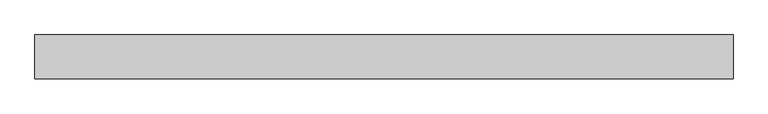
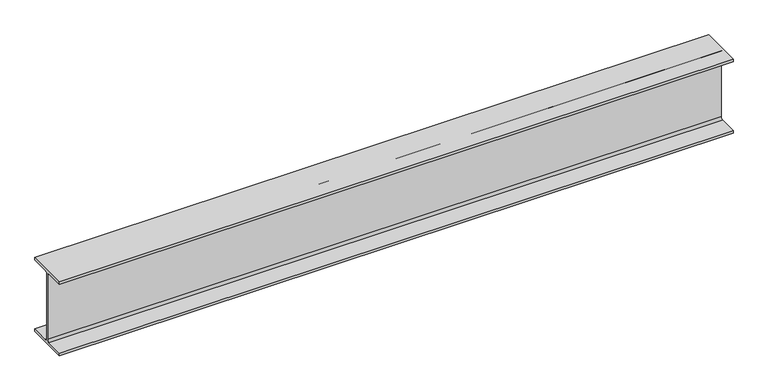
"""IFC4 building model written with IfcOpenShell, lengths in millimetres: beam geometry, Old_Steel Beam_H-KSD3502 : H_SB_ASB_H-194×150x6x9."""

from ifc_helpers import new_model, si_unit, point, frame, frame_2d, origin, place, context, project, spatial, polyline, circle_curve, trimmed, segment, composite_curve, outline, extrude, source, transform, mapped, element, save


def beam_f3b47e3d(model_context):
    return source(origin(), model_context, "Body", "SweptSolid", [
        extrude(outline(composite_curve([segment(polyline([(-82.5, -141.5), (-11.9, -141.5)]), True, "CONTINUOUS"), segment(trimmed(circle_curve(frame_2d((-11.9, -132.6)), 8.9), [point((-11.9, -141.5))], [point((-3.0, -132.6))], True, "CARTESIAN"), True, "CONTINUOUS"), segment(polyline([(-3.0, -132.6), (-3.0, 132.6)]), True, "CONTINUOUS"), segment(trimmed(circle_curve(frame_2d((-11.9, 132.6)), 8.9), [point((-3.0, 132.6))], [point((-11.9, 141.5))], True, "CARTESIAN"), True, "CONTINUOUS"), segment(polyline([(-11.9, 141.5), (-82.5, 141.5), (-82.5, 151.7), (82.5, 151.7), (82.5, 141.5), (11.9, 141.5)]), True, "CONTINUOUS"), segment(trimmed(circle_curve(frame_2d((11.9, 132.6)), 8.9), [point((11.9, 141.5))], [point((3.0, 132.6))], True, "CARTESIAN"), True, "CONTINUOUS"), segment(polyline([(3.0, 132.6), (3.0, -132.6)]), True, "CONTINUOUS"), segment(trimmed(circle_curve(frame_2d((11.9, -132.6)), 8.9), [point((3.0, -132.6))], [point((11.9, -141.5))], True, "CARTESIAN"), True, "CONTINUOUS"), segment(polyline([(11.9, -141.5), (82.5, -141.5), (82.5, -151.7), (-82.5, -151.7), (-82.5, -141.5)]), True, "CONTINUOUS")], self_intersect=False)), frame((-1068.0314701, 0.0, 0.0), z_axis=(1.0, 0.0, 0.0), x_axis=(0.0, 1.0, 0.0)), (0.0, 0.0, 1.0), 2617.0588612),
    ])


if __name__ == "__main__":
    model = new_model("IFC4")
    model_context = context("Model", 3, world=origin())
    ifc_project = project(units=[si_unit("LENGTHUNIT", "METRE", prefix="MILLI")], contexts=[model_context])
    site = spatial("IfcSite", under=ifc_project)
    building = spatial("IfcBuilding", under=site)
    placement = place(None, origin())
    beam_shape = beam_f3b47e3d(model_context)
    element("IfcBeam", 1, ObjectType="Old_Steel Beam_H-KSD3502 : H_SB_ASB_H-194×150x6x9", at=placement, inside=building, context=model_context, shape_type="MappedRepresentation", body=[
        mapped(beam_shape, transform((0.0, 0.0, 0.0), x_axis=(1.0, 0.0, 0.0), y_axis=(0.0, 1.0, 0.0), z_axis=(0.0, 0.0, 1.0))),
    ])
    save(model, "model.ifc")

# Revit data of these elements
# Type "Old_Steel Beam_H-KSD3502 : H_SB_ASB_H-194×150x6x9"
#   Width = 15.0 cm
#   Web Thickness = 0.6 cm
#   Web Fillet = 1.3 cm
#   Warping Constant = 43316.0 cm⁶
#   Torsional Moment of Inertia = 8.622 cm⁴
#   Torsional Modulus = 1.0 cm³
#   Section Area = 39.01 cm²
#   Plastic Modulus weak axis = 104.0 cm³
#   Plastic Modulus strong axis = 309.0 cm³
#   Perimeter = 0.95 m²/m
#   Nominal Weight = 30.60 kgf/m
#   Moment of Inertia weak axis = 507.00 cm⁴
#   Moment of Inertia strong axis = 2690.00 cm⁴
#   Height = 19.4 cm
#   Flange Thickness = 0.9 cm
#   Elastic Modulus weak axis = 67.6 cm³
#   Elastic Modulus strong axis = 277.0 cm³
#   Centroid Vertical = 9.7 cm
#   Centroid Horizontal = 7.5 cm
#   Length [instance default] = 1.5240 m
#   Structural Material [instance default] = Steel, 45-345
#   Assembly Code = ""
# Element 1 (IfcBeam, "Old_Steel Beam_H-KSD3502 : H_SB_ASB_H-194×150x6x9")
#   Structural Material = none
# Materials
#   "Steel, 45-345": class "Metal", colour RGB 189 187 185, transparency 0, Description = "Steel 345 MPa", Cost = 0
